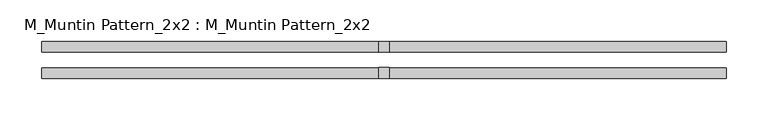
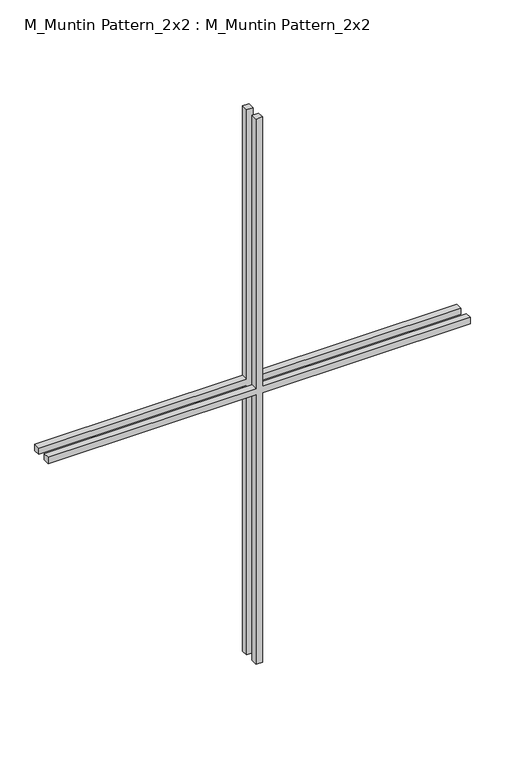
"""IFC4 building model written with IfcOpenShell, lengths in millimetres: proxy geometry, M_Muntin Pattern_2x2 : M_Muntin Pattern_2x2."""

from ifc_helpers import new_model, si_unit, frame, origin, place, context, project, spatial, polyline, outline, extrude, source, transform, mapped, element, save


def m_muntin_pattern_2x2_m_muntin_pattern_2x2_ad852c99(model_context):
    return source(origin(), model_context, "Body", "SweptSolid", [
        extrude(outline(polyline([(568.25, -6.35), (568.25, -411.9), (555.55, -411.9), (555.55, -6.35), (0.0, -6.35), (0.0, 6.35), (555.55, 6.35), (555.55, 411.9), (568.25, 411.9), (568.25, 6.35), (1123.8, 6.35), (1123.8, -6.35), (568.25, -6.35)])), frame((0.0, -22.225, 0.0), z_axis=(0.0, 1.0, 0.0), x_axis=(0.0, 0.0, 1.0)), (0.0, 0.0, 1.0), 12.7),
        extrude(outline(polyline([(568.25, -6.35), (568.25, -411.9), (555.55, -411.9), (555.55, -6.35), (0.0, -6.35), (0.0, 6.35), (555.55, 6.35), (555.55, 411.9), (568.25, 411.9), (568.25, 6.35), (1123.8, 6.35), (1123.8, -6.35), (568.25, -6.35)])), frame((0.0, 9.525, 0.0), z_axis=(0.0, 1.0, 0.0), x_axis=(0.0, 0.0, 1.0)), (0.0, 0.0, 1.0), 12.7),
    ])


if __name__ == "__main__":
    model = new_model("IFC4")
    model_context = context("Model", 3, world=origin())
    ifc_project = project(units=[si_unit("LENGTHUNIT", "METRE", prefix="MILLI")], contexts=[model_context])
    site = spatial("IfcSite", under=ifc_project)
    building = spatial("IfcBuilding", under=site)
    placement = place(None, origin())
    m_muntin_pattern_2x2_m_muntin_pattern_2x2_shape = m_muntin_pattern_2x2_m_muntin_pattern_2x2_ad852c99(model_context)
    element("IfcBuildingElementProxy", 1, Name="M_Muntin Pattern_2x2 : M_Muntin Pattern_2x2", ObjectType="M_Muntin Pattern_2x2 : M_Muntin Pattern_2x2", at=placement, inside=building, context=model_context, shape_type="MappedRepresentation", body=[
        mapped(m_muntin_pattern_2x2_m_muntin_pattern_2x2_shape, transform((0.0, 0.0, 0.0), x_axis=(1.0, 0.0, 0.0), y_axis=(0.0, 1.0, 0.0), z_axis=(0.0, 0.0, 1.0))),
    ])
    save(model, "model.ifc")

# Revit data of these elements
# Type "M_Muntin Pattern_2x2 : M_Muntin Pattern_2x2"
#   Width [instance default] = 1200 mm
#   Thickness = 12.7 mm
#   Height [instance default] = 1200 mm
#   Distance = 19.05 mm
#   Interior Material [instance default] = none
#   Exterior Material [instance default] = none
#   Default Elevation = 0
# Element 1 (IfcBuildingElementProxy, "M_Muntin Pattern_2x2 : M_Muntin Pattern_2x2")
#   Width = 823.8 mm
#   Height = 1123.8 mm
#   Interior Material = Wood - Stained
#   Exterior Material = Clad - White
#   Materials on its faces: "Clad - White", "Wood - Stained"
# Materials
#   "Clad - White": class "Wood", colour RGB 245 245 243, transparency 0, Cost = 0
#   "Wood - Stained": class "Wood", colour RGB 173 132 96, transparency 0, Cost = 0
